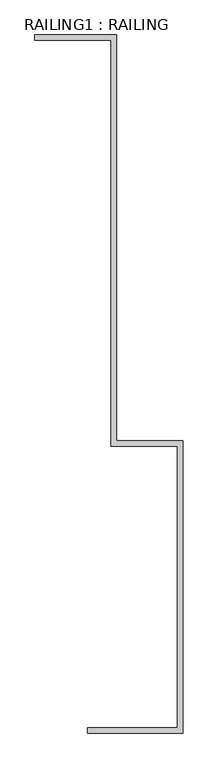
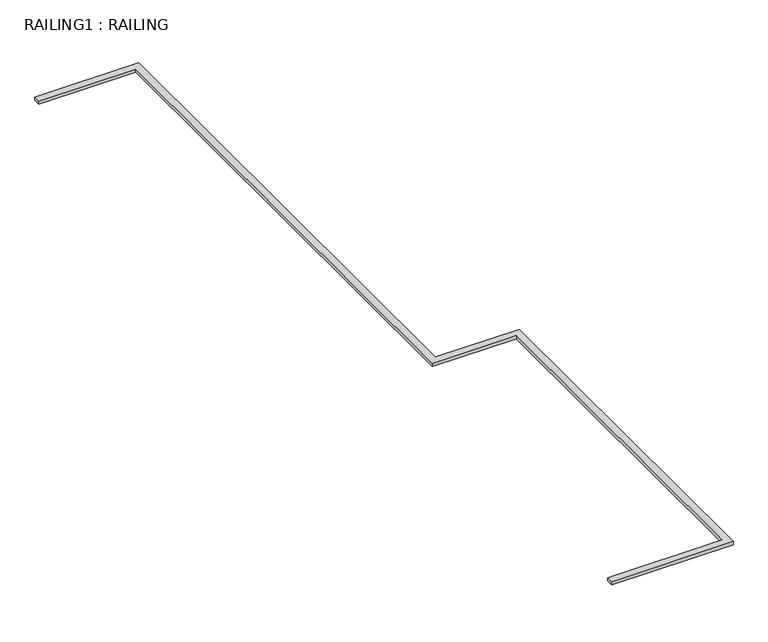
"""IFC4 building model written with IfcOpenShell, lengths in millimetres: proxy geometry, RAILING1 : RAILING."""

from ifc_helpers import new_model, si_unit, frame, origin, place, context, project, spatial, polyline, outline, extrude, source, transform, mapped, element, save


def railing1_railing_f5fd7874(model_context):
    return source(origin(), model_context, "Body", "SweptSolid", [
        extrude(outline(polyline([(16573.5, -9069.3), (16573.5, -9019.3), (17401.9, -9019.3), (17401.9, -6436.6), (16791.7888874, -6436.6), (16791.7888874, -2715.5), (16090.9, -2715.5), (16090.9, -2665.5), (16841.7888874, -2665.5), (16841.7888874, -6386.6), (17451.9, -6386.6), (17451.9, -9069.3), (16573.5, -9069.3)])), frame((0.0, 0.0, 6858.0), z_axis=(0.0, 0.0, 1.0), x_axis=(1.0, 0.0, 0.0)), (0.0, 0.0, 1.0), 25.4370634),
    ])


if __name__ == "__main__":
    model = new_model("IFC4")
    model_context = context("Model", 3, world=origin())
    ifc_project = project(units=[si_unit("LENGTHUNIT", "METRE", prefix="MILLI")], contexts=[model_context])
    site = spatial("IfcSite", under=ifc_project)
    building = spatial("IfcBuilding", under=site)
    placement = place(None, origin())
    railing1_railing_shape = railing1_railing_f5fd7874(model_context)
    element("IfcBuildingElementProxy", 1, Name="RAILING1 : RAILING", ObjectType="RAILING1 : RAILING", at=placement, inside=building, context=model_context, shape_type="MappedRepresentation", body=[
        mapped(railing1_railing_shape, transform((0.0, 0.0, 0.0), x_axis=(1.0, 0.0, 0.0), y_axis=(0.0, 1.0, 0.0), z_axis=(0.0, 0.0, 1.0))),
    ])
    save(model, "model.ifc")

# Revit data of these elements
# Element 1 (IfcBuildingElementProxy, "RAILING1 : RAILING")
#   Materials on its faces: "METAL TEXTURE"
# Materials
#   "METAL TEXTURE": class "Generic", colour RGB 120 120 120, transparency 0, Cost = 0
